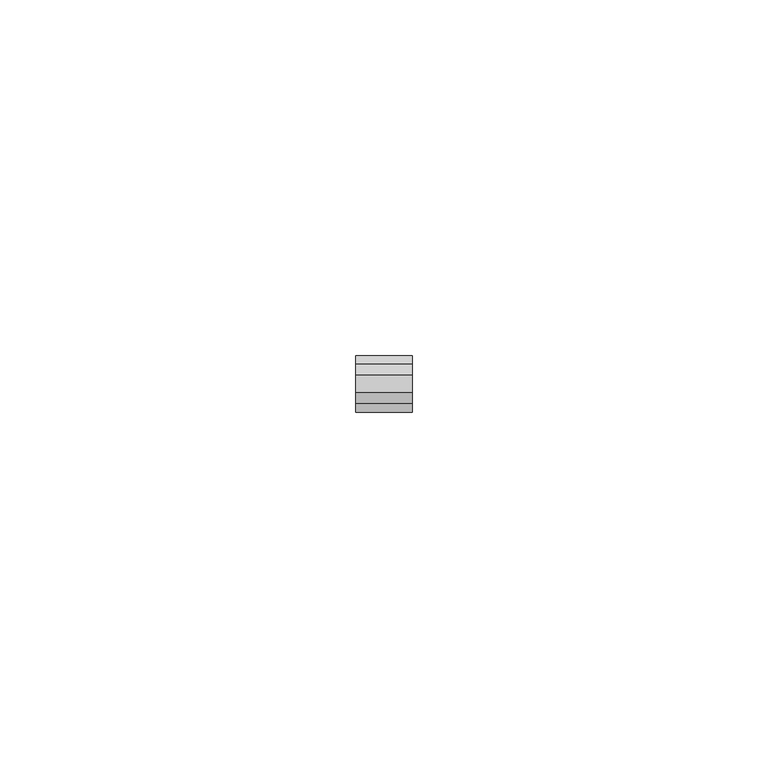
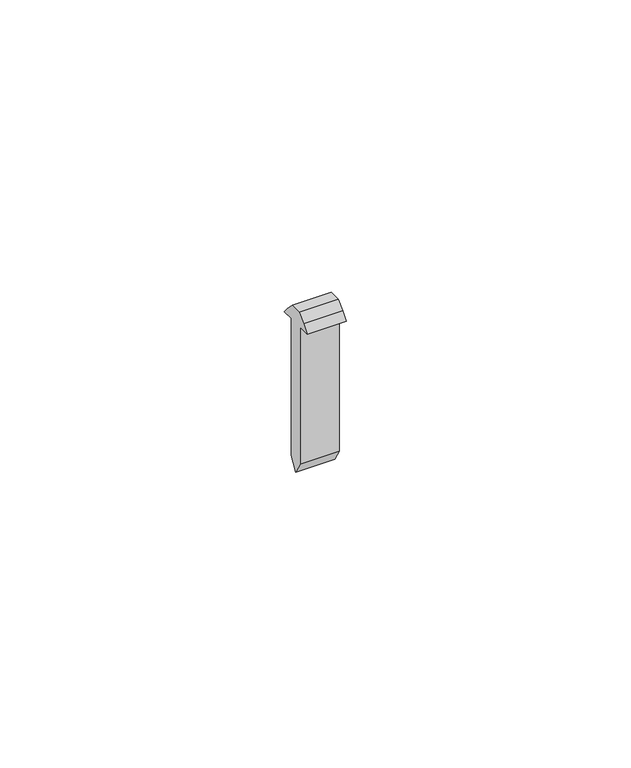
"""IFC4 building model written with IfcOpenShell, lengths in millimetres: proxy geometry, Generic Models 7:Generic Models 1:3:Generic Models 1:3 : Generic Models 7:Generic Models 1:305549:3:Generic Models 1:3:Generic Models 1:3 : Generic Models 7:Generic Models 1:305549:3 : Generic Models 7:Generic Models 1:3:Generic Models 1:3 : Generic Models 7:Generic Models 1:305549:301244:1 : Generic Models 7:Generic Models 1:3:Generic Models 1:3 : Generic Models 7:Generic Models 1:305549:3:Generic Models 1:3:Generic Models 1:3 : Generic Models 7:Generic Models 1:305549:3 : Generic Models 7:Generic Models 1:3:Generic Models 1:3 : Generic Models 7:Generic Models 1:305549:301244:308848."""

from ifc_helpers import new_model, si_unit, frame, origin, place, context, project, spatial, polyline, outline, extrude, source, transform, mapped, element, save


def generic_models_276715c1(model_context):
    return source(origin(), model_context, "Body", "SweptSolid", [
        extrude(outline(polyline([(-1.5875, 0.0), (0.79375, 0.0), (-0.4244455, -1.527058), (-1.9763357, -3.0789482), (-4.3736642, -3.0789482), (-5.9255544, -1.527058), (-7.14375, 0.0), (-4.7625, 0.0), (-4.7625, 29.3030055), (-3.175, 32.0526362), (-1.5875, 29.3030055), (-1.5875, 0.0)])), frame((592641.9179739, -579056.6017699, 38.6090899), z_axis=(1.0, 1.0529910277057297e-12, 5.4343196609352154e-12), x_axis=(1.0529910277288011e-12, -1.0, -4.245492845790196e-12)), (0.0, 0.0, 1.0), 7.9375),
    ])


if __name__ == "__main__":
    model = new_model("IFC4")
    model_context = context("Model", 3, world=origin())
    ifc_project = project(units=[si_unit("LENGTHUNIT", "METRE", prefix="MILLI")], contexts=[model_context])
    site = spatial("IfcSite", under=ifc_project)
    building = spatial("IfcBuilding", under=site)
    placement = place(None, origin())
    generic_models_shape = generic_models_276715c1(model_context)
    element("IfcBuildingElementProxy", 1, Name="Generic Models 7:Generic Models 1:3:Generic Models 1:3 : Generic Models 7:Generic Models 1:305549:3:Generic Models 1:3:Generic Models 1:3 : Generic Models 7:Generic Models 1:305549:3 : Generic Models 7:Generic Models 1:3:Generic Models 1:3 : Generic Models 7:Generic Models 1:305549:301244:1 : Generic Models 7:Generic Models 1:3:Generic Models 1:3 : Generic Models 7:Generic Models 1:305549:3:Generic Models 1:3:Generic Models 1:3 : Generic Models 7:Generic Models 1:305549:3 : Generic Models 7:Generic Models 1:3:Generic Models 1:3 : Generic Models 7:Generic Models 1:305549:301244:308848", ObjectType="Generic Models 7:Generic Models 1:3:Generic Models 1:3 : Generic Models 7:Generic Models 1:305549:3:Generic Models 1:3:Generic Models 1:3 : Generic Models 7:Generic Models 1:305549:3 : Generic Models 7:Generic Models 1:3:Generic Models 1:3 : Generic Models 7:Generic Models 1:305549:301244:1 : Generic Models 7:Generic Models 1:3:Generic Models 1:3 : Generic Models 7:Generic Models 1:305549:3:Generic Models 1:3:Generic Models 1:3 : Generic Models 7:Generic Models 1:305549:3 : Generic Models 7:Generic Models 1:3:Generic Models 1:3 : Generic Models 7:Generic Models 1:305549:301244:308848", at=placement, inside=building, context=model_context, shape_type="MappedRepresentation", body=[
        mapped(generic_models_shape, transform((0.0, 0.0, 0.0), x_axis=(1.0, 0.0, 0.0), y_axis=(0.0, 1.0, 0.0), z_axis=(0.0, 0.0, 1.0))),
    ])
    save(model, "model.ifc")

# Revit data of these elements
# Type "Generic Models 7:Generic Models 1:3:Generic Models 1:3 : Generic Models 7:Generic Models 1:305549:3:Generic Models 1:3:Generic Models 1:3 : Generic Models 7:Generic Models 1:305549:3 : Generic Models 7:Generic Models 1:3:Generic Models 1:3 : Generic Models 7:Generic Models 1:305549:301244:1 : Generic Models 7:Generic Models 1:3:Generic Models 1:3 : Generic Models 7:Generic Models 1:305549:3:Generic Models 1:3:Generic Models 1:3 : Generic Models 7:Generic Models 1:305549:3 : Generic Models 7:Generic Models 1:3:Generic Models 1:3 : Generic Models 7:Generic Models 1:305549:301244:308848"
#   NameOverride = "Generic Models 7:Generic Models 1:3:Generic Models 1:3 : Generic Models 7:Generic Models 1:305549:3:Generic Models 1:3:Generic Models 1:3 : Generic Models 7:Generic Models 1:305549:3 : Generic Models 7:Generic Models 1:3:Generic Models 1:3 : Generic Models 7:Generic Models 1:305549:301244:308848"
#   ObjectTypeOverride = "Generic Models 1:3:Generic Models 1:3 : Generic Models 7:Generic Models 1:305549:3 : Generic Models 7:Generic Models 1:3:Generic Models 1:3 : Generic Models 7:Generic Models 1:305549:301244"
#   Reference = "Generic Models 1"
#   Tag = "308848"
# Element 1 (IfcBuildingElementProxy, "Generic Models 7:Generic Models 1:3:Generic Models 1:3 : Generic Models 7:Generic Models 1:305549:3:Generic Models 1:3:Generic Models 1:3 : Generic Models 7:Generic Models 1:305549:3 : Generic Models 7:Generic Models 1:3:Generic Models 1:3 : Generic Models 7:Generic Models 1:305549:301244:1 : Generic Models 7:Generic Models 1:3:Generic Models 1:3 : Generic Models 7:Generic Models 1:305549:3:Generic Models 1:3:Generic Models 1:3 : Generic Models 7:Generic Models 1:305549:3 : Generic Models 7:Generic Models 1:3:Generic Models 1:3 : Generic Models 7:Generic Models 1:305549:301244:308848")
#   Materials on its faces: "FASTENERS (T.B.D)"
# Materials
#   "FASTENERS (T.B.D)": class "Generic", colour RGB 120 120 120, transparency 0, Cost = 0
